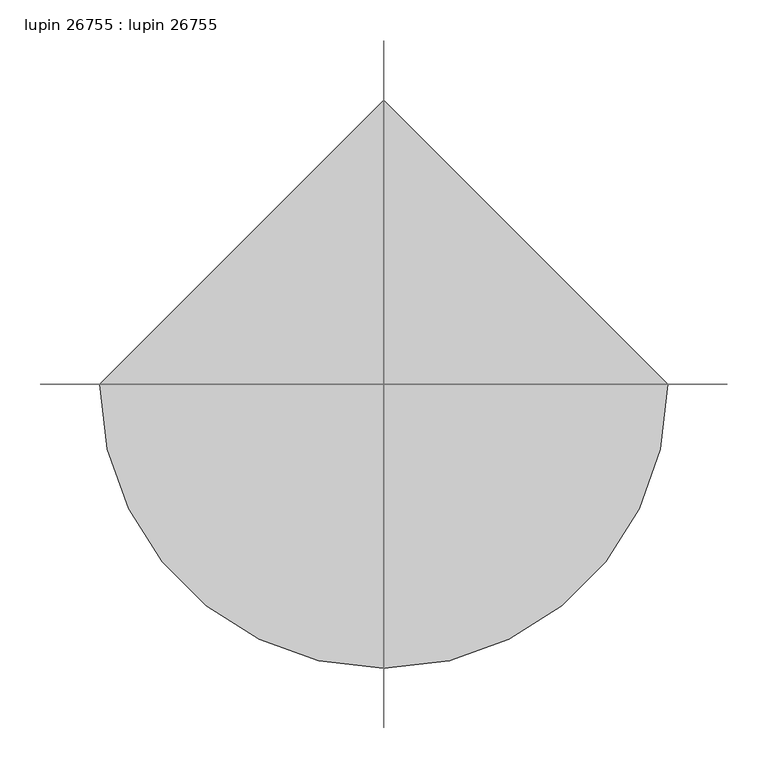
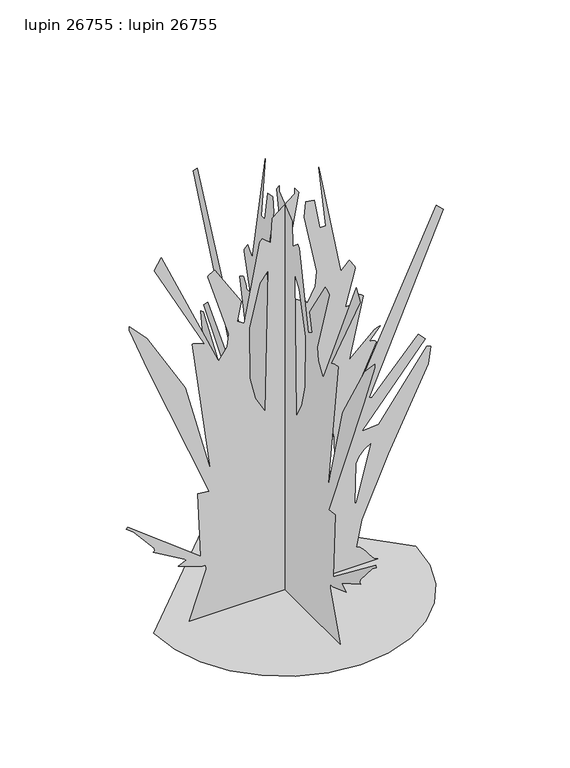
"""IFC4 building model written with IfcOpenShell, lengths in millimetres: proxy geometry, lupin 26755 : lupin 26755."""

from ifc_helpers import new_model, si_unit, origin, place, context, project, spatial, triangles, source, transform, mapped, element, save


def lupin_26755_lupin_26755_1db73bb0(model_context):
    return source(origin(), model_context, "Body", "Tessellation", [
        triangles([(-351.9469769, 0.0, 0.0), (-342.6429663, -80.6431063, 0.0), (-316.1457464, -154.7010223, 0.0), (-274.573611, -220.0515756, 0.0), (-220.0515756, -274.573611, 0.0), (-154.700768, -316.1457464, 0.0), (-80.6431063, -342.6429663, 0.0), (1.54e-05, -351.9469769, 0.0), (80.6431063, -342.6429663, 0.0), (154.7010223, -316.1457464, 0.0), (220.0515756, -274.573611, 0.0), (274.573611, -220.0515756, 0.0), (316.1457464, -154.700768, 0.0), (342.6429663, -80.6431063, 0.0), (351.9469769, 3.08e-05, 0.0), (-4.62e-05, 351.9469769, 0.0), (150.6720804, -0.0015947, 851.9910187), (173.2724542, -0.0015961, 874.5918921), (188.3394669, -0.0015947, 851.9910187), (188.5203062, -0.0015944, 847.0684994), (161.9722718, -0.0015884, 746.5202036), (177.0392664, -0.0015884, 746.5202036), (178.9694175, -0.0015886, 750.284436), (180.6039107, -0.0015889, 754.0461977), (182.1639718, -0.0015891, 757.8054159), (183.8723704, -0.0015893, 761.5671049), (185.9508409, -0.0015895, 765.3339535), (188.6214083, -0.0015898, 769.1058163), (192.1062791, -0.00159, 772.8878529), (193.2812801, -0.00159, 772.4611347), (195.5106317, -0.0015899, 771.3080074), (198.4649026, -0.0015898, 769.6264967), (201.8143893, -0.0015897, 767.6173897), (205.2296787, -0.0015896, 765.4761686), (208.3815575, -0.0015894, 763.4010046), (210.9401041, -0.0015893, 761.5874525), (173.2724542, -0.0015792, 592.0833366), (240.700733, -0.0015829, 654.2395718), (250.6943454, -0.0015832, 659.6218014), (256.1408516, -0.0015833, 659.8859568), (226.0070987, -0.0015812, 625.984683), (228.5658996, -0.0015812, 626.1598904), (231.7175241, -0.0015812, 625.7001801), (235.1327953, -0.0015812, 624.7324339), (238.4825545, -0.0015811, 623.3938528), (241.4365711, -0.001581, 621.8114639), (243.6659227, -0.0015809, 620.1197794), (244.8409236, -0.0015808, 618.4509859), (180.8060786, -0.0015725, 479.0814042), (184.572909, -0.0015725, 479.0814042), (406.8108882, -0.0016005, 949.9256659), (425.6449857, -0.0015994, 931.0915684), (226.0070987, -0.0015718, 467.7809675), (233.5407231, -0.0015716, 464.0141553), (357.8448363, -0.0015797, 599.6169611), (376.6763904, -0.0015785, 580.7828636), (207.1732737, -0.0015664, 377.3799811), (252.3745481, -0.0015666, 381.1467934), (380.4432026, -0.0015772, 558.1819902), (391.7436393, -0.001577, 554.4177215), (384.6443633, -0.0015741, 506.8385036), (278.1600926, -0.0015612, 289.3386073), (206.7572381, -0.0015515, 126.6752076), (192.1062791, -0.0015471, 53.437713), (201.6487926, -0.0015469, 49.4892894), (210.1163717, -0.0015464, 41.8553304), (217.9390592, -0.0015458, 32.010051), (225.5471159, -0.0015452, 21.427562), (233.3697852, -0.0015446, 11.5823576), (241.8373824, -0.0015442, 3.9483989), (251.3798959, -0.0015439, 1.66e-05), (-256.5091613, -0.001544, 0.4898205), (-211.4973739, -0.0015518, 132.0554297), (-212.2487088, -0.0015525, 144.4635658), (-222.2372343, -0.0015525, 143.8397394), (-286.2728424, -0.0015538, 166.4403676), (-263.6719508, -0.0015545, 177.7405681), (-354.0729735, -0.0015577, 230.4752126), (-348.9472326, -0.0015578, 232.5839138), (-351.022433, -0.0015583, 241.0403199), (-406.3257797, -0.0015621, 305.3939318), (-425.6424422, -0.0015631, 320.8777614), (-421.87563, -0.0015633, 324.6445736), (-226.0037922, -0.0015543, 173.9740102), (-233.5374348, -0.0015651, 354.7790714), (-203.4034275, -0.0015648, 351.0122592), (-366.5443417, -0.0015886, 750.3606668), (-417.7760619, -0.0015966, 882.9891266), (-418.1088178, -0.0015972, 893.4259169), (-370.8775801, -0.0015942, 843.3371864), (-268.1575782, -0.0015837, 667.2316566), (-199.6365971, -0.0015682, 407.5119355), (-248.6044294, -0.0015907, 784.1883259), (-246.3971695, -0.0015907, 784.2213181), (-242.3227634, -0.0015906, 783.3755121), (-236.9745433, -0.0015905, 781.8490065), (-230.9453692, -0.0015904, 779.8398268), (-224.8285369, -0.0015903, 777.5436733), (-219.2169245, -0.0015901, 775.1611879), (-214.7036098, -0.00159, 772.8878529), (-350.306125, -0.0016053, 1029.028759), (-331.4720638, -0.0016071, 1059.1632568), (-180.8027903, -0.0015866, 716.3881765), (-177.0359781, -0.0015864, 712.6214006), (-155.1577168, -0.0015883, 744.8692142), (-150.1099781, -0.0015904, 779.1769312), (-207.1702397, -0.0016012, 961.2260662), (-205.9949844, -0.0016013, 963.0370749), (-203.7656147, -0.0016014, 965.1147823), (-194.0468402, -0.0016018, 970.9440777), (-190.8949614, -0.0016019, 972.0972776), (-188.3364148, -0.0016019, 972.5265392), (-116.7679544, -0.0015952, 859.5246431), (-128.0681458, -0.001592, 806.7891993), (-109.2343208, -0.0015913, 795.4887989), (-67.8001221, -0.0016041, 1010.1946615), (-60.2664931, -0.0016046, 1017.728286), (-37.6658604, -0.0016035, 998.8941885), (-33.8993003, -0.0016075, 1066.6968813), (26.3689732, -0.0016104, 1115.6629332), (26.3689732, -0.0016113, 1130.7301821), (37.6691624, -0.0016104, 1115.6629332), (2.9836067, -0.0015988, 921.19319), (5.2254839, -0.0015953, 862.2830503), (21.4607608, -0.0015927, 818.4376162), (56.5029828, -0.0015916, 799.2555748), (60.269795, -0.0015911, 791.7219503), (81.2288264, -0.0015936, 833.4109028), (86.0914021, -0.0015961, 874.8052511), (51.7460784, -0.0016059, 1039.955781), (56.5029828, -0.0016084, 1081.7615868), (79.10362, -0.0016082, 1077.9948109), (94.1706237, -0.0016032, 995.1274126), (109.237373, -0.0016032, 995.1274126), (90.4038023, -0.0016136, 1168.3983044), (-67.325905, -0.0015972, 893.4183592), (-96.1172708, -0.0015902, 776.6851501), (-94.9783414, -0.0015817, 633.9373953), (-79.6923831, -0.001578, 571.2782112), (-52.7331184, -0.0015752, 524.2831873), (-45.1994894, -0.001599, 923.5579439), (109.237373, -0.0015608, 283.2096027), (135.6048224, -0.0015619, 302.0436639), (131.8382554, -0.0015682, 407.5119355), (211.912919, -0.0015632, 322.7039944), (198.2078507, -0.0015623, 307.9059877), (189.9752137, -0.0015612, 290.5146256), (188.3394669, -0.0015547, 181.5073803), (192.1062791, -0.0015545, 177.7405681), (232.2618404, -0.0015639, 335.5792259), (0.0016106, 150.6687739, 851.9910187), (0.0016109, 173.269402, 874.5918921), (0.00161, 188.3364148, 851.9910187), (0.0016099, 188.5169997, 847.0684994), (0.0016073, 161.9689653, 746.5202036), (0.001607, 177.0362324, 746.5202036), (0.0016071, 178.9663653, 750.284436), (0.0016072, 180.6006042, 754.0461977), (0.0016073, 182.1609196, 757.8054159), (0.0016074, 183.8693182, 761.5671049), (0.0016075, 185.9478069, 765.3339535), (0.0016076, 188.6183561, 769.1058163), (0.0016076, 192.103227, 772.8878529), (0.0016076, 193.2782279, 772.4611347), (0.0016075, 195.5075795, 771.3080074), (0.0016074, 198.4615962, 769.6264967), (0.0016073, 201.8113554, 767.6173897), (0.0016072, 205.2266265, 765.4761686), (0.0016071, 208.378251, 763.4010046), (0.001607, 210.937052, 761.5874525), (0.0016025, 173.269402, 592.0833366), (0.0016033, 240.6974266, 654.2395718), (0.0016034, 250.6910389, 659.6218014), (0.0016033, 256.1383082, 659.8859568), (0.0016027, 226.0040465, 625.984683), (0.0016027, 228.5625931, 626.1598904), (0.0016026, 231.7142176, 625.7001801), (0.0016026, 235.1297431, 624.7324339), (0.0016025, 238.479248, 623.3938528), (0.0016024, 241.4332646, 621.8114639), (0.0016023, 243.6626162, 620.1197794), (0.0016022, 244.8378715, 618.4509859), (0.001599, 180.8027903, 479.0814042), (0.001599, 184.5696025, 479.0814042), (0.0016097, 406.8083447, 949.9256659), (0.0016088, 425.6424422, 931.0915684), (0.001598, 226.0040465, 467.7809675), (0.0015978, 233.5374348, 464.0141553), (0.0016, 357.8397858, 599.6169611), (0.0015991, 376.6738469, 580.7828636), (0.0015956, 207.1702397, 377.3799811), (0.001595, 252.3712416, 381.1467934), (0.0015984, 380.4406591, 558.1845337), (0.0015981, 391.7410958, 554.4177215), (0.0015968, 384.6418199, 506.8385036), (0.0015919, 278.1575492, 289.3386073), (0.0015881, 206.7539316, 126.6752076), (0.0015862, 192.103227, 53.437713), (0.0015859, 201.6454861, 49.4892894), (0.0015856, 210.1130652, 41.8553304), (0.0015851, 217.936007, 32.010051), (0.0015847, 225.5438094, 21.427587), (0.0015843, 233.3664787, 11.5823837), (0.001584, 241.8343303, 3.9483989), (0.0015837, 251.3765894, 2.41e-05), (0.0015913, -256.51423, 0.4898434), (0.0015945, -211.5006804, 132.0554297), (0.0015949, -212.2519971, 144.4635658), (0.001595, -222.2402864, 143.8397394), (0.0015967, -286.2753676, 166.4403676), (0.0015967, -263.6744943, 177.7405681), (0.0015996, -354.0780241, 230.4752126), (0.0015996, -348.9497761, 232.5839138), (0.0015999, -351.0249764, 241.0403199), (0.0016026, -406.3308303, 305.3939318), (0.0016033, -425.6449857, 320.8777614), (0.0016034, -421.8781734, 324.6445736), (0.001596, -226.0070987, 173.9740102), (0.0016015, -233.5404688, 354.7790714), (0.0016009, -203.4064615, 351.0122592), (0.0016153, -366.5468851, 750.3606668), (0.00162, -417.7786054, 882.9891266), (0.0016203, -418.1113612, 893.4259169), (0.0016181, -370.8801235, 843.3371864), (0.0016113, -268.1626651, 667.2316566), (0.0016026, -199.6396492, 407.5119355), (0.0016145, -248.6077359, 784.1883259), (0.0016145, -246.4002216, 784.2213181), (0.0016144, -242.3260699, 783.3755121), (0.0016143, -236.9775955, 781.8490065), (0.0016141, -230.9484032, 779.8398268), (0.001614, -224.8318434, 777.5436733), (0.0016138, -219.2199766, 775.1611879), (0.0016137, -214.7069163, 772.8878529), (0.0016233, -350.3112119, 1029.028759), (0.0016239, -331.4771507, 1059.1632568), (0.0016115, -180.8060786, 716.3881765), (0.0016113, -177.0392664, 712.6214006), (0.001612, -155.1607508, 744.8692142), (0.0016129, -150.1132755, 779.1769312), (0.0016192, -207.1732737, 961.2260662), (0.0016192, -205.9982728, 963.0396183), (0.0016192, -203.7689212, 965.1147823), (0.0016193, -194.0498742, 970.9466211), (0.0016193, -190.8979953, 972.0998211), (0.0016192, -188.3394669, 972.5265392), (0.0016148, -116.7709974, 859.5246431), (0.0016134, -128.0714432, 806.7891993), (0.0016128, -109.2376273, 795.4887989), (0.0016186, -67.8031697, 1010.1946615), (0.0016187, -60.269795, 1017.728286), (0.0016178, -37.6691624, 998.8941885), (0.0016197, -33.9023479, 1066.6968813), (0.0016203, 26.3656713, 1115.6629332), (0.0016207, 26.3656713, 1130.7301821), (0.0016201, 37.6661148, 1115.6629332), (0.0016148, 2.9804319, 921.19319), (0.0016131, 5.2223085, 862.2830503), (0.0016115, 21.4575588, 818.4376162), (0.0016104, 56.4999352, 799.2555748), (0.0016101, 60.2664931, 791.7219503), (0.0016111, 81.225529, 833.4109028), (0.0016122, 86.0883499, 874.8052511), (0.0016177, 51.7430263, 1039.955781), (0.0016188, 56.4999352, 1081.7615868), (0.0016184, 79.1003135, 1077.9948109), (0.0016157, 94.1673172, 995.1274126), (0.0016155, 109.2340665, 995.1274126), (0.0016209, 90.4007593, 1168.3983044), (0.0016151, -67.329207, 893.4183592), (0.001612, -96.120323, 776.6851501), (0.0016077, -94.9816388, 633.9373953), (0.0016057, -79.6956896, 571.2782112), (0.0016039, -52.736166, 524.2831873), (0.0016156, -45.202537, 923.5579439), (0.0015943, 109.2340665, 283.2096027), (0.0015944, 135.6017703, 302.0436639), (0.0015976, 131.834958, 407.5119355), (0.0015939, 211.9098669, 322.7039944), (0.0015937, 198.2045624, 307.9059877), (0.0015933, 189.9719254, 290.5146256), (0.00159, 188.3364148, 181.5073803), (0.0015899, 192.103227, 177.7405681), (0.001594, 232.2587883, 335.5792259)], [[15, 16, 1], [14, 15, 1], [14, 1, 2], [13, 14, 2], [13, 2, 3], [13, 3, 4], [12, 13, 4], [11, 12, 4], [11, 4, 5], [11, 5, 6], [11, 6, 7], [11, 7, 8], [11, 8, 9], [11, 9, 10], [144, 142, 18], [134, 135, 17], [70, 71, 72], [120, 121, 122], [17, 18, 142], [140, 17, 142], [88, 89, 90], [69, 70, 72], [39, 40, 41], [38, 39, 41], [37, 38, 41], [75, 76, 77], [77, 78, 79], [68, 69, 72], [101, 102, 103], [100, 101, 103], [67, 68, 72], [66, 67, 72], [65, 66, 72], [64, 65, 72], [147, 148, 143], [50, 51, 52], [50, 52, 53], [119, 120, 122], [118, 119, 122], [142, 143, 148], [84, 85, 86], [64, 72, 73], [92, 93, 94], [92, 94, 95], [92, 95, 96], [92, 96, 97], [92, 97, 98], [92, 98, 99], [92, 99, 100], [92, 100, 103], [92, 103, 104], [81, 82, 83], [81, 83, 84], [80, 81, 84], [79, 80, 84], [77, 79, 84], [75, 77, 84], [130, 131, 132], [130, 132, 133], [54, 55, 56], [54, 56, 57], [63, 64, 73], [87, 88, 90], [87, 90, 91], [87, 91, 92], [86, 87, 92], [74, 75, 84], [63, 73, 74], [116, 117, 118], [115, 116, 118], [118, 122, 123], [53, 54, 57], [50, 53, 57], [59, 60, 61], [58, 59, 61], [58, 61, 62], [57, 58, 62], [49, 50, 57], [146, 147, 143], [146, 143, 144], [145, 146, 144], [150, 145, 144], [133, 134, 17], [130, 133, 17], [129, 130, 17], [128, 129, 17], [128, 17, 140], [127, 128, 140], [28, 29, 30], [35, 36, 37], [34, 35, 37], [33, 34, 37], [32, 33, 37], [31, 32, 37], [30, 31, 37], [28, 30, 37], [27, 28, 37], [26, 27, 37], [25, 26, 37], [24, 25, 37], [23, 24, 37], [22, 23, 37], [21, 22, 37], [111, 112, 113], [110, 111, 113], [109, 110, 113], [108, 109, 113], [107, 108, 113], [107, 113, 114], [106, 107, 114], [63, 74, 84], [63, 84, 86], [63, 86, 92], [47, 48, 49], [46, 47, 49], [45, 46, 49], [44, 45, 49], [43, 44, 49], [42, 43, 49], [41, 42, 49], [37, 41, 49], [63, 92, 104], [105, 106, 114], [105, 114, 115], [126, 127, 140], [125, 126, 140], [125, 140, 141], [124, 125, 141], [123, 124, 141], [118, 123, 141], [118, 141, 136], [115, 118, 136], [115, 136, 137], [105, 115, 137], [104, 105, 137], [104, 137, 138], [104, 138, 139], [18, 19, 20], [18, 20, 21], [144, 18, 21], [144, 21, 37], [144, 37, 49], [144, 49, 57], [150, 144, 57], [150, 57, 62], [149, 150, 62], [149, 62, 63], [148, 149, 63], [142, 148, 63], [104, 139, 140], [63, 104, 140], [63, 140, 142], [278, 276, 152], [268, 269, 151], [204, 205, 206], [254, 255, 256], [151, 152, 276], [274, 151, 276], [222, 223, 224], [203, 204, 206], [173, 174, 175], [172, 173, 175], [171, 172, 175], [209, 210, 211], [211, 212, 213], [202, 203, 206], [235, 236, 237], [234, 235, 237], [201, 202, 206], [200, 201, 206], [199, 200, 206], [198, 199, 206], [281, 282, 277], [184, 185, 186], [184, 186, 187], [253, 254, 256], [252, 253, 256], [276, 277, 282], [218, 219, 220], [198, 206, 207], [226, 227, 228], [226, 228, 229], [226, 229, 230], [226, 230, 231], [226, 231, 232], [226, 232, 233], [226, 233, 234], [226, 234, 237], [226, 237, 238], [215, 216, 217], [215, 217, 218], [214, 215, 218], [213, 214, 218], [211, 213, 218], [209, 211, 218], [264, 265, 266], [264, 266, 267], [188, 189, 190], [188, 190, 191], [197, 198, 207], [221, 222, 224], [221, 224, 225], [221, 225, 226], [220, 221, 226], [208, 209, 218], [197, 207, 208], [250, 251, 252], [249, 250, 252], [252, 256, 257], [187, 188, 191], [184, 187, 191], [193, 194, 195], [192, 193, 195], [192, 195, 196], [191, 192, 196], [183, 184, 191], [280, 281, 277], [280, 277, 278], [279, 280, 278], [284, 279, 278], [267, 268, 151], [264, 267, 151], [263, 264, 151], [262, 263, 151], [262, 151, 274], [261, 262, 274], [162, 163, 164], [169, 170, 171], [168, 169, 171], [167, 168, 171], [166, 167, 171], [165, 166, 171], [164, 165, 171], [162, 164, 171], [161, 162, 171], [160, 161, 171], [159, 160, 171], [158, 159, 171], [157, 158, 171], [156, 157, 171], [155, 156, 171], [245, 246, 247], [244, 245, 247], [243, 244, 247], [242, 243, 247], [241, 242, 247], [241, 247, 248], [240, 241, 248], [197, 208, 218], [197, 218, 220], [197, 220, 226], [181, 182, 183], [180, 181, 183], [179, 180, 183], [178, 179, 183], [177, 178, 183], [176, 177, 183], [175, 176, 183], [171, 175, 183], [197, 226, 238], [239, 240, 248], [239, 248, 249], [260, 261, 274], [259, 260, 274], [259, 274, 275], [258, 259, 275], [257, 258, 275], [252, 257, 275], [252, 275, 270], [249, 252, 270], [249, 270, 271], [239, 249, 271], [238, 239, 271], [238, 271, 272], [238, 272, 273], [152, 153, 154], [152, 154, 155], [278, 152, 155], [278, 155, 171], [278, 171, 183], [278, 183, 191], [284, 278, 191], [284, 191, 196], [283, 284, 196], [283, 196, 197], [282, 283, 197], [276, 282, 197], [238, 273, 274], [197, 238, 274], [197, 274, 276]], closed=False),
    ])


if __name__ == "__main__":
    model = new_model("IFC4")
    model_context = context("Model", 3, world=origin())
    ifc_project = project(units=[si_unit("LENGTHUNIT", "METRE", prefix="MILLI")], contexts=[model_context])
    site = spatial("IfcSite", under=ifc_project)
    building = spatial("IfcBuilding", under=site)
    placement = place(None, origin())
    lupin_26755_lupin_26755_shape = lupin_26755_lupin_26755_1db73bb0(model_context)
    element("IfcBuildingElementProxy", 1, Name="lupin 26755 : lupin 26755", ObjectType="lupin 26755 : lupin 26755", at=placement, inside=building, context=model_context, shape_type="MappedRepresentation", body=[
        mapped(lupin_26755_lupin_26755_shape, transform((0.0, 0.0, 0.0), x_axis=(1.0, 0.0, 0.0), y_axis=(0.0, 1.0, 0.0), z_axis=(0.0, 0.0, 1.0))),
    ])
    save(model, "model.ifc")

# Revit data of these elements
# Type "lupin 26755 : lupin 26755"
#   built-in parameter 1005195 = "RPC-16-G2M4-C67X-C72M-U000-ST1L-LVER-AU"
#   Height = 0
